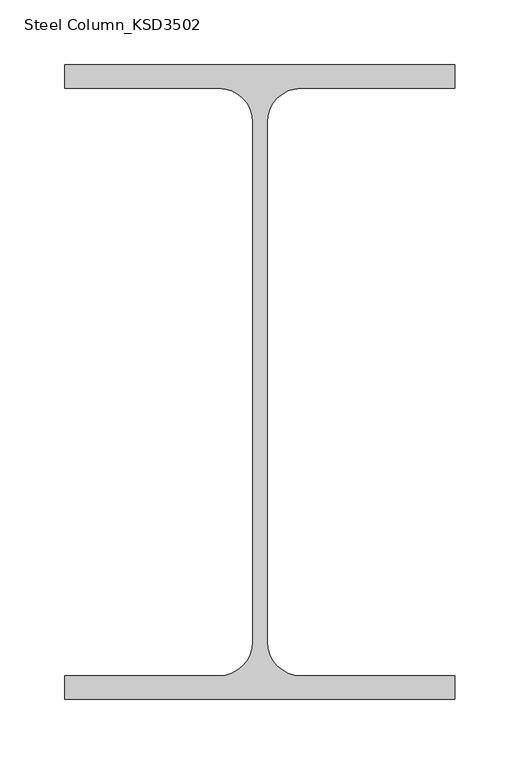
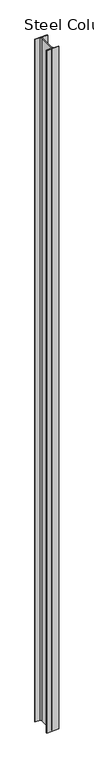
"""IFC4 building model written with IfcOpenShell, lengths in millimetres: column geometry, Steel Column_KSD3502 : H_SC_ASC_H-488×300x11x18."""

from ifc_helpers import new_model, si_unit, point, frame, frame_2d, origin, place, context, project, spatial, polyline, circle_curve, trimmed, segment, composite_curve, outline, extrude, source, transform, mapped, element, save


def steel_column_ksd3502_c3fe6796(model_context):
    return source(origin(), model_context, "Body", "SweptSolid", [
        extrude(outline(composite_curve([segment(polyline([(150.0, 244.0), (150.0, 226.0), (31.5, 226.0)]), True, "CONTINUOUS"), segment(trimmed(circle_curve(frame_2d((31.5, 200.0)), 26.0), [point((31.5, 226.0))], [point((5.5, 200.0))], True, "CARTESIAN"), True, "CONTINUOUS"), segment(polyline([(5.5, 200.0), (5.5, -200.0)]), True, "CONTINUOUS"), segment(trimmed(circle_curve(frame_2d((31.5, -200.0)), 26.0), [point((5.5, -200.0))], [point((31.5, -226.0))], True, "CARTESIAN"), True, "CONTINUOUS"), segment(polyline([(31.5, -226.0), (150.0, -226.0), (150.0, -244.0), (-150.0, -244.0), (-150.0, -226.0), (-31.5, -226.0)]), True, "CONTINUOUS"), segment(trimmed(circle_curve(frame_2d((-31.5, -200.0)), 26.0), [point((-31.5, -226.0))], [point((-5.5, -200.0))], True, "CARTESIAN"), True, "CONTINUOUS"), segment(polyline([(-5.5, -200.0), (-5.5, 200.0)]), True, "CONTINUOUS"), segment(trimmed(circle_curve(frame_2d((-31.5, 200.0)), 26.0), [point((-5.5, 200.0))], [point((-31.5, 226.0))], True, "CARTESIAN"), True, "CONTINUOUS"), segment(polyline([(-31.5, 226.0), (-150.0, 226.0), (-150.0, 244.0), (150.0, 244.0)]), True, "CONTINUOUS")], self_intersect=False)), frame((0.0, 0.0, 685.9720055), z_axis=(0.0, 0.0, 1.0), x_axis=(1.0, 0.0, 0.0)), (0.0, 0.0, 1.0), 17514.0),
    ])


if __name__ == "__main__":
    model = new_model("IFC4")
    model_context = context("Model", 3, world=origin())
    ifc_project = project(units=[si_unit("LENGTHUNIT", "METRE", prefix="MILLI")], contexts=[model_context])
    site = spatial("IfcSite", under=ifc_project)
    building = spatial("IfcBuilding", under=site)
    placement = place(None, origin())
    steel_column_ksd3502_shape = steel_column_ksd3502_c3fe6796(model_context)
    element("IfcColumn", 1, ObjectType="Steel Column_KSD3502 : H_SC_ASC_H-488×300x11x18", at=placement, inside=building, context=model_context, shape_type="MappedRepresentation", body=[
        mapped(steel_column_ksd3502_shape, transform((0.0, 0.0, 0.0), x_axis=(1.0, 0.0, 0.0), y_axis=(0.0, 1.0, 0.0), z_axis=(0.0, 0.0, 1.0))),
    ])
    save(model, "model.ifc")

# Revit data of these elements
# Type "Steel Column_KSD3502 : H_SC_ASC_H-488×300x11x18"
#   Width = 30.0 cm
#   Web Thickness = 1.1 cm
#   Web Fillet = 2.6 cm
#   Warping Constant = 4473230.0 cm⁶
#   Torsional Moment of Inertia = 137.492 cm⁴
#   Section Area = 163.5 cm²
#   Plastic Modulus weak axis = 830.0 cm³
#   Plastic Modulus strong axis = 3230.0 cm³
#   Perimeter = 1.27 m²/m
#   Nominal Weight = 128.00 kgf/m
#   Moment of Inertia weak axis = 8110.00 cm⁴
#   Moment of Inertia strong axis = 71000.00 cm⁴
#   Height = 48.8 cm
#   Flange Thickness = 1.8 cm
#   Elastic Modulus weak axis = 541.0 cm³
#   Elastic Modulus strong axis = 2910.0 cm³
#   Centroid Vertical = 24.4 cm
#   Centroid Horizontal = 15.0 cm
#   Bolt Spacing = 13.97 cm
#   Structural Material [instance default] = Steel, 45-345
#   Section Name Key = ""
#   Assembly Code = ""
# Element 1 (IfcColumn, "Steel Column_KSD3502 : H_SC_ASC_H-488×300x11x18")
#   Structural Material = A03AD029-00005_Anchor Bolt (Installation only)_M24
#   Materials on its faces: "A03AD029-00005_Anchor Bolt (Installation only)_M24"
# Materials
#   "Steel, 45-345": class "Metal", colour RGB 189 187 185, transparency 0, Description = "Steel 345 MPa", Cost = 0
#   "A03AD029-00005_Anchor Bolt (Installation only)_M24": class "Unassigned", colour RGB 84 83 81, transparency 0, Cost = 0
